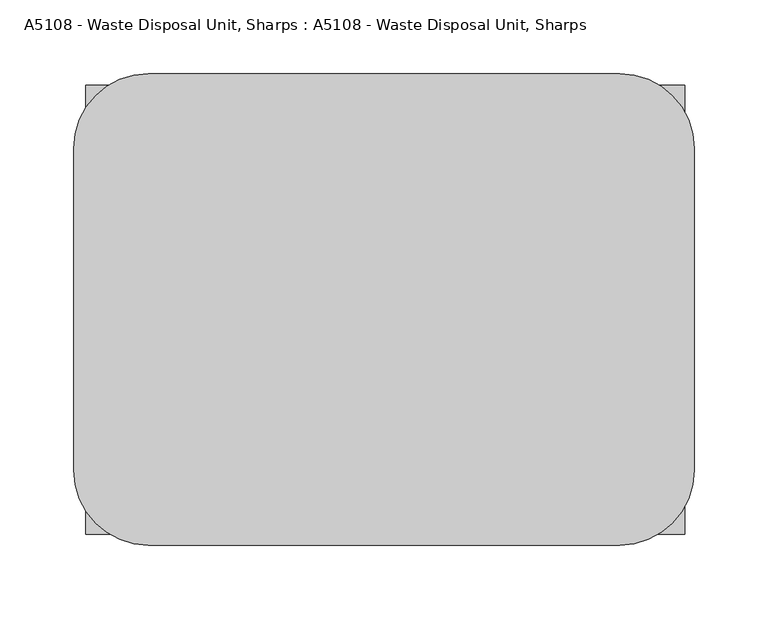
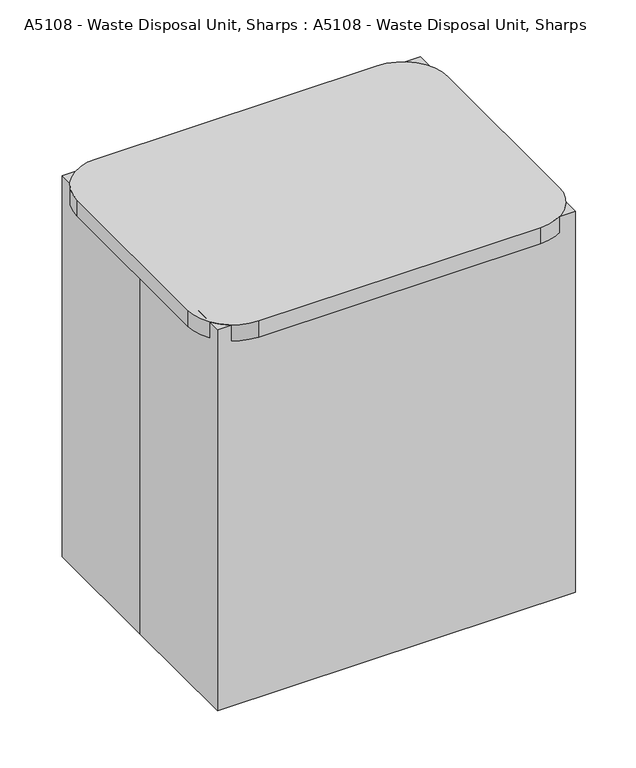
"""IFC4 building model written with IfcOpenShell, lengths in millimetres: proxy geometry, A5108 - Waste Disposal Unit, Sharps : A5108 - Waste Disposal Unit, Sharps."""

import ifcopenshell
import ifcopenshell.guid

model = None  # the IFC model being written
_history = None  # IfcOwnerHistory: only IFC2X3 demands one
_inside = {}  # id of a spatial element -> (the spatial element, [elements in it])
_under = {}  # id of a project, library or spatial element -> (it, [spatial elements below it])
_declared = {}  # id of a project -> (the project, [libraries it declares])
_typed = {}  # id of a type object -> (the type object, [elements of that type])
_made_of = {}  # id of a material, layer set ... -> (it, [elements and type objects made of it])


def new_model(schema):
    """Start an empty IFC model of exactly this schema.

    Asked for "IFC4X3", IfcOpenShell would pick the latest addendum, in which some entities
    have other attributes; the version numbers below select the first issue.
    IFC2X3 requires an IfcOwnerHistory on every rooted entity: one is made here for all.
    """
    global model, _history
    if schema == "IFC4X3":
        model = ifcopenshell.file(schema_version=(4, 3, 0, 0))
    else:
        model = ifcopenshell.file(schema=schema)
    _inside.clear()
    _under.clear()
    _declared.clear()
    _typed.clear()
    _made_of.clear()
    _history = None
    if model.schema == "IFC2X3":
        org = make("IfcOrganization", Name="unknown")
        user = make(
            "IfcPersonAndOrganization",
            ThePerson=make("IfcPerson", FamilyName="unknown"),
            TheOrganization=org,
        )
        app = make(
            "IfcApplication",
            ApplicationDeveloper=org,
            Version="unknown",
            ApplicationFullName="unknown",
            ApplicationIdentifier="unknown",
        )
        _history = make(
            "IfcOwnerHistory",
            OwningUser=user,
            OwningApplication=app,
            ChangeAction="ADDED",
            CreationDate=0,
        )
    return model


def make(cls, **values):
    """One entity of the class cls with the attributes given. An attribute that is None is left unset."""
    return model.create_entity(
        cls, **{name: value for name, value in values.items() if value is not None}
    )


def rooted(cls, **values):
    """An entity with a GlobalId (a new one), such as an element, a storey or a relation."""
    return make(cls, GlobalId=ifcopenshell.guid.new(), OwnerHistory=_history, **values)


def si_unit(unit_type, name, prefix=None):
    """IfcSIUnit, for example si_unit("LENGTHUNIT", "METRE", prefix="MILLI")."""
    return make("IfcSIUnit", UnitType=unit_type, Prefix=prefix, Name=name)


def assignment(units):
    """IfcUnitAssignment: the units of a project."""
    return None if units is None else make("IfcUnitAssignment", Units=units)


def point(xyz):
    """IfcCartesianPoint."""
    return None if xyz is None else make("IfcCartesianPoint", Coordinates=xyz)


def direction(xyz):
    """IfcDirection."""
    return None if xyz is None else make("IfcDirection", DirectionRatios=xyz)


def frame(location, z_axis=None, x_axis=None):
    """IfcAxis2Placement3D, a coordinate frame: its origin and axes. An axis left out is left unset."""
    return make(
        "IfcAxis2Placement3D",
        Location=point(location),
        Axis=direction(z_axis),
        RefDirection=direction(x_axis),
    )


def frame_2d(location, x_axis=None):
    """IfcAxis2Placement2D, a coordinate frame in the plane: its origin and x axis."""
    return make(
        "IfcAxis2Placement2D", Location=point(location), RefDirection=direction(x_axis)
    )


def origin():
    """The frame at (0, 0, 0) with its axes left unset."""
    return frame((0.0, 0.0, 0.0))


def origin_with_axes():
    """The frame at (0, 0, 0) with the z axis (0, 0, 1) and the x axis (1, 0, 0) written out."""
    return frame((0.0, 0.0, 0.0), z_axis=(0.0, 0.0, 1.0), x_axis=(1.0, 0.0, 0.0))


def place(relative_to, where):
    """IfcLocalPlacement: puts the frame where relative to a parent placement (None: the world)."""
    return make(
        "IfcLocalPlacement", PlacementRelTo=relative_to, RelativePlacement=where
    )


def context(
    kind, dimensions, precision=None, world=None, true_north=None, identifier=None
):
    """IfcGeometricRepresentationContext, for example the 3D "Model" context."""
    return make(
        "IfcGeometricRepresentationContext",
        ContextIdentifier=identifier,
        ContextType=kind,
        CoordinateSpaceDimension=dimensions,
        Precision=precision,
        WorldCoordinateSystem=world,
        TrueNorth=true_north,
    )


def project(units=None, contexts=None):
    """IfcProject with its units and contexts."""
    return rooted(
        "IfcProject",
        Name="project",
        RepresentationContexts=contexts,
        UnitsInContext=assignment(units),
    )


def spatial(cls, under=None, at=None, **own):
    """A site, building, storey or space (cls), placed at a placement, below another one or the project."""
    s = rooted(cls, ObjectPlacement=at, **own)
    if under is not None:
        _under.setdefault(under.id(), (under, []))[1].append(s)
    return s


def polyline(points):
    """IfcPolyline through the points."""
    return make("IfcPolyline", Points=[point(p) for p in points])


def circle_curve(where, radius):
    """IfcCircle in the frame where."""
    return make("IfcCircle", Position=where, Radius=radius)


def trimmed(basis, trim1, trim2, sense, master):
    """IfcTrimmedCurve: the piece of a basis curve between two trims."""
    return make(
        "IfcTrimmedCurve",
        BasisCurve=basis,
        Trim1=trim1,
        Trim2=trim2,
        SenseAgreement=sense,
        MasterRepresentation=master,
    )


def segment(curve, same_sense, transition):
    """IfcCompositeCurveSegment."""
    return make(
        "IfcCompositeCurveSegment",
        Transition=transition,
        SameSense=same_sense,
        ParentCurve=curve,
    )


def composite_curve(segments, self_intersect=None):
    """IfcCompositeCurve: segments joined end to end."""
    return make("IfcCompositeCurve", Segments=segments, SelfIntersect=self_intersect)


def outline(outer, holes=None, kind="AREA"):
    """IfcArbitraryClosedProfileDef: a profile drawn as a closed curve; with holes, ...WithVoids."""
    if holes is None:
        return make("IfcArbitraryClosedProfileDef", ProfileType=kind, OuterCurve=outer)
    return make(
        "IfcArbitraryProfileDefWithVoids",
        ProfileType=kind,
        OuterCurve=outer,
        InnerCurves=holes,
    )


def extrude(swept, where, along, depth):
    """IfcExtrudedAreaSolid: the profile swept, set in the frame where, extruded along a direction by depth."""
    return make(
        "IfcExtrudedAreaSolid",
        SweptArea=swept,
        Position=where,
        ExtrudedDirection=direction(along),
        Depth=depth,
    )


def shape(context_of_items, identifier, shape_type, items):
    """IfcShapeRepresentation: the items that make up one representation, for example the "Body"."""
    return make(
        "IfcShapeRepresentation",
        ContextOfItems=context_of_items,
        RepresentationIdentifier=identifier,
        RepresentationType=shape_type,
        Items=items,
    )


def source(mapping_origin, context_of_items, identifier, shape_type, items):
    """IfcRepresentationMap: a shape defined once, which mapped items show again and again."""
    return make(
        "IfcRepresentationMap",
        MappingOrigin=mapping_origin,
        MappedRepresentation=shape(context_of_items, identifier, shape_type, items),
    )


def transform(
    local_origin,
    x_axis=None,
    y_axis=None,
    z_axis=None,
    scale=None,
    scale2=None,
    scale3=None,
    uniform=True,
):
    """IfcCartesianTransformationOperator3D, or its non-uniform kind. x_axis, y_axis, z_axis: its Axis1, 2, 3."""
    if uniform:
        return make(
            "IfcCartesianTransformationOperator3D",
            Axis1=direction(x_axis),
            Axis2=direction(y_axis),
            LocalOrigin=point(local_origin),
            Scale=scale,
            Axis3=direction(z_axis),
        )
    return make(
        "IfcCartesianTransformationOperator3DnonUniform",
        Axis1=direction(x_axis),
        Axis2=direction(y_axis),
        LocalOrigin=point(local_origin),
        Scale=scale,
        Axis3=direction(z_axis),
        Scale2=scale2,
        Scale3=scale3,
    )


def mapped(mapping_source, mapping_target):
    """IfcMappedItem: shows the shape of a source again, moved by a transform."""
    return make(
        "IfcMappedItem", MappingSource=mapping_source, MappingTarget=mapping_target
    )


def made_of(thing, what):
    """Note that an element or type object is made of a material, layer set ...; save() writes the relation."""
    if what is not None:
        _made_of.setdefault(what.id(), (what, []))[1].append(thing)
    return thing


def element(
    cls,
    number,
    at=None,
    inside=None,
    cuts=None,
    type_object=None,
    material=None,
    context=None,
    identifier="Body",
    shape_type=None,
    held_by="IfcProductDefinitionShape",
    body=None,
    shapes=None,
    **own,
):
    """One element of the class cls, such as IfcWall. Its Tag is "e" and its number.

    at: its placement. inside: the storey or other place that contains it. cuts: it is an
    opening in that element (IfcRelVoidsElement). A single representation is given by context,
    identifier, shape_type and body (its items); several are given by shapes. held_by: the class
    of the entity that holds the representations. save() writes the other relations.
    """
    e = rooted(cls, Tag="e%d" % number, ObjectPlacement=at, **own)
    if body is not None:
        shapes = [shape(context, identifier, shape_type, body)]
    if shapes is not None:
        e.Representation = make(held_by, Representations=shapes)
    if inside is not None:
        _inside.setdefault(inside.id(), (inside, []))[1].append(e)
    if cuts is not None:
        rooted(
            "IfcRelVoidsElement", RelatingBuildingElement=cuts, RelatedOpeningElement=e
        )
    if type_object is not None:
        _typed.setdefault(type_object.id(), (type_object, []))[1].append(e)
    return made_of(e, material)


def aggregate(whole, parts):
    """IfcRelAggregates: a whole, such as a stair, and the parts it consists of."""
    return rooted("IfcRelAggregates", RelatingObject=whole, RelatedObjects=parts)


def save(model, path):
    """Write the relations noted so far, then the file.

    IfcRelAggregates (storeys below a building ...), IfcRelContainedInSpatialStructure (elements
    in a storey), IfcRelDefinesByType, IfcRelAssociatesMaterial and IfcRelDeclares: one each for
    every whole, place, type object, material and project.
    """
    for whole, parts in _under.values():
        aggregate(whole, parts)
    for where, things in _inside.values():
        rooted(
            "IfcRelContainedInSpatialStructure",
            RelatedElements=things,
            RelatingStructure=where,
        )
    for kind, things in _typed.values():
        rooted("IfcRelDefinesByType", RelatedObjects=things, RelatingType=kind)
    for what, things in _made_of.values():
        rooted("IfcRelAssociatesMaterial", RelatedObjects=things, RelatingMaterial=what)
    for by, libraries in _declared.values():
        rooted("IfcRelDeclares", RelatingContext=by, RelatedDefinitions=libraries)
    model.write(path)


def plane_surface(at):
    """IfcPlane: the flat surface through the origin of the frame at, square to its z axis."""
    return make("IfcPlane", Position=at)


def spline_surface(u_degree, v_degree, points, u_multiplicities, v_multiplicities, u_knots, v_knots, weights=None):
    """IfcBSplineSurfaceWithKnots; with weights, IfcRationalBSplineSurfaceWithKnots. points: one row for each step in u."""
    own = dict(
        UDegree=u_degree,
        VDegree=v_degree,
        ControlPointsList=[[point(p) for p in row] for row in points],
        SurfaceForm="UNSPECIFIED",
        UClosed=False,
        VClosed=False,
        SelfIntersect=False,
        UMultiplicities=u_multiplicities,
        VMultiplicities=v_multiplicities,
        UKnots=u_knots,
        VKnots=v_knots,
        KnotSpec="UNSPECIFIED",
    )
    if weights is None:
        return make("IfcBSplineSurfaceWithKnots", **own)
    return make("IfcRationalBSplineSurfaceWithKnots", WeightsData=weights, **own)


def advanced_brep(points, edges, surfaces, faces):
    """IfcAdvancedBrep: a solid bounded by faces that lie on surfaces and meet in shared edges.

    An edge is (start, end): straight between two places in points (the first is 0);
    or (start, end, curve); or (start, end, curve, False) where it runs against its curve.
    A face is (place in surfaces, loops), or (place, loops, False) where it looks against
    its surface's normal. A loop lists edges by number (the first is 1), with a minus sign
    where the edge is run from its end to its start. The first loop is the outer one.
    """
    corners = [point(p) for p in points]
    vertices = [make("IfcVertexPoint", VertexGeometry=c) for c in corners]
    made = []
    for start, end, *more in edges:
        made.append(
            make(
                "IfcEdgeCurve",
                EdgeStart=vertices[start],
                EdgeEnd=vertices[end],
                EdgeGeometry=more[0] if more else make("IfcPolyline", Points=[corners[start], corners[end]]),
                SameSense=more[1] if len(more) > 1 else True,
            )
        )
    hull = []
    for where, loops, *sense in faces:
        bounds = []
        for j, loop in enumerate(loops):
            ring = [make("IfcOrientedEdge", EdgeElement=made[abs(k) - 1], Orientation=k > 0) for k in loop]
            bounds.append(
                make(
                    "IfcFaceOuterBound" if j == 0 else "IfcFaceBound",
                    Bound=make("IfcEdgeLoop", EdgeList=ring),
                    Orientation=True,
                )
            )
        hull.append(make("IfcAdvancedFace", Bounds=bounds, FaceSurface=surfaces[where], SameSense=sense[0] if sense else True))
    return make("IfcAdvancedBrep", Outer=make("IfcClosedShell", CfsFaces=hull))


def a5108_waste_disposal_unit_sharps_a5108_waste_disposal_unit_e3dd660a(model_context):
    return source(origin(), model_context, "Body", "SolidModel", [
        extrude(outline(composite_curve([segment(trimmed(circle_curve(frame_2d((159.003917, 109.5639811)), 50.8), [point((159.003917, 160.3639811))], [point((209.803917, 109.5639811))], False, "CARTESIAN"), True, "CONTINUOUS"), segment(polyline([(209.803917, 109.5639811), (209.803917, -108.8679249)]), True, "CONTINUOUS"), segment(trimmed(circle_curve(frame_2d((159.003917, -108.8679249)), 50.8), [point((209.803917, -108.8679249))], [point((159.003917, -159.6679249))], False, "CARTESIAN"), True, "CONTINUOUS"), segment(polyline([(159.003917, -159.6679249), (-160.7733941, -159.6679249)]), True, "CONTINUOUS"), segment(trimmed(circle_curve(frame_2d((-160.7733941, -108.8679249)), 50.8), [point((-160.7733941, -159.6679249))], [point((-211.5733941, -108.8679249))], False, "CARTESIAN"), True, "CONTINUOUS"), segment(polyline([(-211.5733941, -108.8679249), (-211.5733941, 109.5639811)]), True, "CONTINUOUS"), segment(trimmed(circle_curve(frame_2d((-160.7733941, 109.5639811)), 50.8), [point((-211.5733941, 109.5639811))], [point((-160.7733941, 160.3639811))], False, "CARTESIAN"), True, "CONTINUOUS"), segment(polyline([(-160.7733941, 160.3639811), (159.003917, 160.3639811)]), True, "CONTINUOUS")], self_intersect=False)), frame((0.0, 0.0, 437.8974387), z_axis=(0.0, 0.0, 1.0), x_axis=(1.0, 0.0, 0.0)), (0.0, 0.0, 1.0), 19.3025613),
        advanced_brep(
        [(141.0040588, 113.3386173, 0.0), (166.4040588, 87.9386173, 0.0), (166.4040588, -76.2, 0.0), (141.0040588, -101.6, 0.0), (-145.3589273, -101.6, 0.0), (-170.7589273, -76.2, 0.0), (-170.7589273, 87.9386173, 0.0), (-145.3589273, 113.3386173, 0.0), (152.4, 152.4, 437.8974387), (-152.4, 152.4, 437.8974387), (-203.2, 101.6, 437.8974387), (-203.2, -101.6, 437.8974387), (-152.4, -152.4, 437.8974387), (152.4, -152.4, 437.8974387), (203.2, -101.6, 437.8974387), (203.2, 101.6, 437.8974387)],
        [
            (0, 1, circle_curve(frame((141.0040588, 87.9386173, 0.0), z_axis=(0.0, 0.0, -1.0), x_axis=(1.0, 0.0, 0.0)), 25.4)),
            (1, 2),
            (2, 3, circle_curve(frame((141.0040588, -76.2, 0.0), z_axis=(0.0, 0.0, -1.0), x_axis=(1.0, 0.0, 0.0)), 25.4)),
            (3, 4),
            (4, 5, circle_curve(frame((-145.3589273, -76.2, 0.0), z_axis=(0.0, 0.0, -1.0), x_axis=(1.0, 0.0, 0.0)), 25.4)),
            (5, 6),
            (6, 7, circle_curve(frame((-145.3589273, 87.9386173, 0.0), z_axis=(0.0, 0.0, -1.0), x_axis=(1.0, 0.0, 0.0)), 25.4)),
            (7, 0),
            (8, 9),
            (9, 10, circle_curve(frame((-152.4, 101.6, 437.8974387), z_axis=(0.0, 0.0, 1.0), x_axis=(1.0, 0.0, 0.0)), 50.8)),
            (10, 11),
            (11, 12, circle_curve(frame((-152.4, -101.6, 437.8974387), z_axis=(0.0, 0.0, 1.0), x_axis=(1.0, 0.0, 0.0)), 50.8)),
            (12, 13),
            (13, 14, circle_curve(frame((152.4, -101.6, 437.8974387), z_axis=(0.0, 0.0, 1.0), x_axis=(1.0, 0.0, 0.0)), 50.8)),
            (14, 15),
            (15, 8, circle_curve(frame((152.4, 101.6, 437.8974387), z_axis=(0.0, 0.0, 1.0), x_axis=(1.0, 0.0, 0.0)), 50.8)),
            (8, 0),
            (7, 9),
            (6, 10),
            (5, 11),
            (4, 12),
            (3, 13),
            (2, 14),
            (1, 15),
        ],
        [
            plane_surface(frame((-2.1774343, 5.8693086, 0.0), z_axis=(0.0, 0.0, -1.0), x_axis=(-1.0, 0.0, 0.0))),
            plane_surface(frame((0.0, 0.0, 437.8974387), z_axis=(0.0, 0.0, 1.0), x_axis=(-1.0, 0.0, 0.0))),
            plane_surface(frame((0.0, 152.4, 437.8974387), z_axis=(0.0, 0.9960450767748678, -0.08884933895391632), x_axis=(1.0, 0.0, 0.0))),
            spline_surface(2, 1, [[(-203.2, 101.6, 437.8974387), (-170.7589273, 87.9386173, 0.0)], [(-203.19999999999996, 152.39999999999998, 437.8974387), (-170.75892729999998, 113.33861730000001, 0.0)], [(-152.4, 152.4, 437.8974387), (-145.3589273, 113.3386173, 0.0)]], [3, 3], [2, 2], [0.0, 1.0], [0.0, 1.0], weights=[[1.0, 1.0], [0.7071067811865478, 0.7071067811865478], [1.0, 1.0]]),
            plane_surface(frame((-203.2, 0.0, 437.8974387), z_axis=(-0.9972670455010029, 0.0, -0.07388125579401594), x_axis=(0.0, 1.0, 0.0))),
            spline_surface(2, 1, [[(-152.4, -152.4, 437.8974387), (-145.3589273, -101.6, 0.0)], [(-203.20000000000002, -152.40000000000003, 437.8974387), (-170.75892729999998, -101.60000000000001, 0.0)], [(-203.2, -101.6, 437.8974387), (-170.7589273, -76.2, 0.0)]], [3, 3], [2, 2], [0.0, 1.0], [0.0, 1.0], weights=[[1.0, 1.0], [0.7071067811865474, 0.7071067811865474], [1.0, 1.0]]),
            plane_surface(frame((0.0, -152.4, 437.8974387), z_axis=(0.0, -0.9933381345616705, -0.11523606391030766), x_axis=(-1.0, 0.0, 0.0))),
            spline_surface(2, 1, [[(203.2, -101.6, 437.8974387), (166.4040588, -76.2, 0.0)], [(203.19999999999996, -152.39999999999998, 437.8974387), (166.40405879999997, -101.60000000000001, 0.0)], [(152.4, -152.4, 437.8974387), (141.0040588, -101.6, 0.0)]], [3, 3], [2, 2], [0.0, 1.0], [0.0, 1.0], weights=[[1.0, 1.0], [0.7071067811865478, 0.7071067811865478], [1.0, 1.0]]),
            plane_surface(frame((203.2, 0.0, 437.8974387), z_axis=(0.9964881773157944, 0.0, -0.08373358029993602), x_axis=(0.0, -1.0, 0.0))),
            spline_surface(2, 1, [[(152.4, 152.4, 437.8974387), (141.0040588, 113.3386173, 0.0)], [(203.20000000000002, 152.40000000000003, 437.8974387), (166.40405879999997, 113.33861730000001, 0.0)], [(203.2, 101.6, 437.8974387), (166.4040588, 87.9386173, 0.0)]], [3, 3], [2, 2], [0.0, 1.0], [0.0, 1.0], weights=[[1.0, 1.0], [0.7071067811865474, 0.7071067811865474], [1.0, 1.0]]),
        ],
        [
            (0, [[1, 2, 3, 4, 5, 6, 7, 8]]),
            (1, [[9, 10, 11, 12, 13, 14, 15, 16]]),
            (2, [[-9, 17, -8, 18]]),
            (3, [[-10, -18, -7, 19]]),
            (4, [[-11, -19, -6, 20]]),
            (5, [[-12, -20, -5, 21]]),
            (6, [[-13, -21, -4, 22]]),
            (7, [[-14, -22, -3, 23]]),
            (8, [[-15, -23, -2, 24]]),
            (9, [[-16, -24, -1, -17]]),
        ],
    ),
        extrude(outline(polyline([(-203.2, 152.4), (203.2, 152.4), (203.2, -152.4), (-203.2, -152.4), (-203.2, 0.0), (-203.2, 152.4)])), origin_with_axes(), (0.0, 0.0, 1.0), 457.2),
    ])


if __name__ == "__main__":
    model = new_model("IFC4")
    model_context = context("Model", 3, world=origin())
    ifc_project = project(units=[si_unit("LENGTHUNIT", "METRE", prefix="MILLI")], contexts=[model_context])
    site = spatial("IfcSite", under=ifc_project)
    building = spatial("IfcBuilding", under=site)
    placement = place(None, origin())
    a5108_waste_disposal_unit_sharps_a5108_waste_disposal_unit_shape = a5108_waste_disposal_unit_sharps_a5108_waste_disposal_unit_e3dd660a(model_context)
    element("IfcBuildingElementProxy", 1, Name="A5108 - Waste Disposal Unit, Sharps : A5108 - Waste Disposal Unit, Sharps", ObjectType="A5108 - Waste Disposal Unit, Sharps : A5108 - Waste Disposal Unit, Sharps", at=placement, inside=building, context=model_context, shape_type="MappedRepresentation", body=[
        mapped(a5108_waste_disposal_unit_sharps_a5108_waste_disposal_unit_shape, transform((0.0, 0.0, 0.0), x_axis=(1.0, 0.0, 0.0), y_axis=(0.0, 1.0, 0.0), z_axis=(0.0, 0.0, 1.0))),
    ])
    save(model, "model.ifc")

# Revit data of these elements
# Type "A5108 - Waste Disposal Unit, Sharps : A5108 - Waste Disposal Unit, Sharps"
#   Watts2 = "0"
#   Watts1 = "0"
#   Unit_Issue = "EA"
#   UTIL_6_Misc = "-"
#   UTIL_5_NonMedGas = "-"
#   UTIL_4_MiscGas = "-"
#   UTIL_3_MedGas = "-"
#   UTIL_2_Elec = "-"
#   UTIL_1_WaterDrain = "-"
#   Nomenclature = "Waste Disposal Unit, Sharps"
#   NSN = "6530"
#   Location [instance default] = ""
#   JSN = "A5108"
#   Fund_Source_VA = "-"
#   Fund_Source_Navy = "-"
#   Fund_Source_Army = "-"
#   Fund_Source_AF = "-"
#   ELEC_Volts2 = "0"
#   ELEC_Volts1 = "0"
#   ELEC_Phase2 = "0"
#   ELEC_Phase1 = "0"
#   ELEC_HertzSwitch = "0"
#   ELEC_HertzDependent = "0"
#   ELEC_Hertz = "0"
#   ELEC_Amps2 = "0"
#   ELEC_Amps1 = "0"
#   DetailDescription = "A container for collecting and transporting syringes and other sharps for decontamination and disposal. Available in 2 gallon and 8 gallon with locking rotor. Complies with OSHA regulations for handling sharps."
#   CAT_VA = "C"
#   CAT_Navy = "C"
#   CAT_IHS = "-"
#   CAT_Army = "C"
#   CAT_AF = "C"
#   BTUperhour = "0"
#   Weight_IP = 2
#   DIM_Width_IP = 1' - 4"
#   DIM_Height_IP = 1' - 6"
#   DIM_Depth_IP = 1' - 0"
# Element 1 (IfcBuildingElementProxy, "A5108 - Waste Disposal Unit, Sharps : A5108 - Waste Disposal Unit, Sharps")
#   Materials on its faces: "EquipSpace"
# Materials
#   "EquipSpace": class "Unassigned", colour RGB 221 217 195, transparency 0.5
